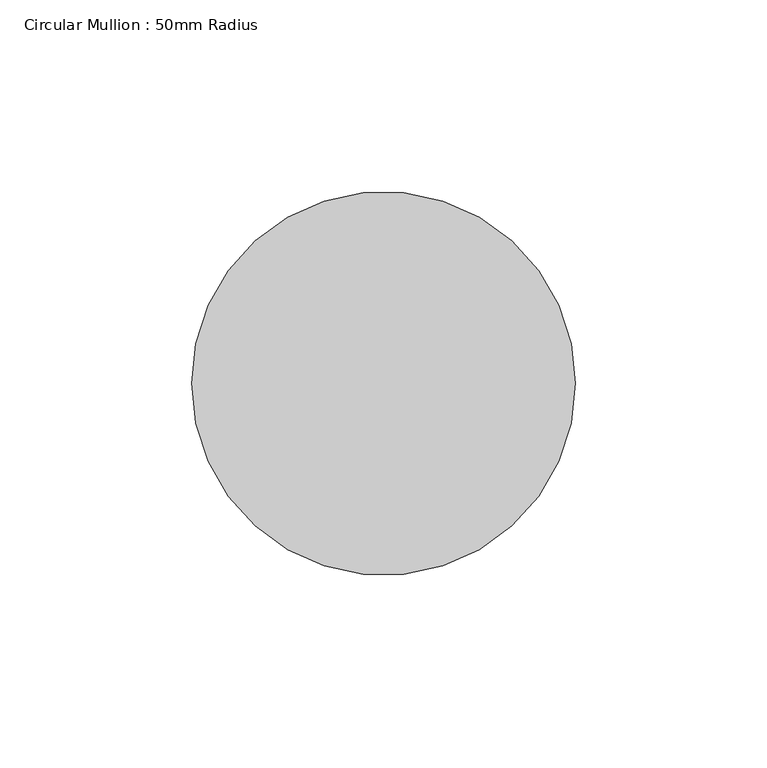
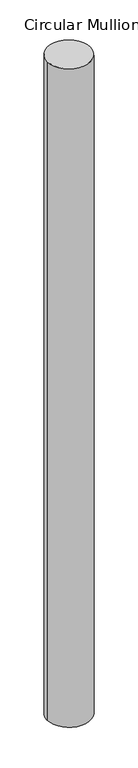
"""IFC4 building model written with IfcOpenShell, lengths in millimetres: member geometry, Circular Mullion : 50mm Radius."""

from ifc_helpers import new_model, si_unit, point, frame, origin, origin_2d, place, context, project, spatial, circle_curve, trimmed, segment, composite_curve, outline, extrude, source, transform, mapped, element, save


def circular_mullion_50mm_radius_9371b420(model_context):
    return source(origin(), model_context, "Body", "SweptSolid", [
        extrude(outline(composite_curve([segment(trimmed(circle_curve(origin_2d(), 50.0), [point((50.0, 0.0))], [point((-50.0, 0.0))], False, "CARTESIAN"), True, "CONTINUOUS"), segment(trimmed(circle_curve(origin_2d(), 50.0), [point((-50.0, 0.0))], [point((50.0, 0.0))], False, "CARTESIAN"), True, "CONTINUOUS")], self_intersect=False)), frame((0.0, 0.0, -1608.4946912), z_axis=(0.0, 0.0, 1.0), x_axis=(1.0, 0.0, 0.0)), (0.0, 0.0, 1.0), 1608.4946912),
    ])


if __name__ == "__main__":
    model = new_model("IFC4")
    model_context = context("Model", 3, world=origin())
    ifc_project = project(units=[si_unit("LENGTHUNIT", "METRE", prefix="MILLI")], contexts=[model_context])
    site = spatial("IfcSite", under=ifc_project)
    building = spatial("IfcBuilding", under=site)
    placement = place(None, origin())
    circular_mullion_50mm_radius_shape = circular_mullion_50mm_radius_9371b420(model_context)
    element("IfcMember", 1, ObjectType="Circular Mullion : 50mm Radius", at=placement, inside=building, context=model_context, shape_type="MappedRepresentation", body=[
        mapped(circular_mullion_50mm_radius_shape, transform((0.0, 0.0, 0.0), x_axis=(1.0, 0.0, 0.0), y_axis=(0.0, 1.0, 0.0), z_axis=(0.0, 0.0, 1.0))),
    ])
    save(model, "model.ifc")

# Revit data of these elements
# Type "Circular Mullion : 50mm Radius"
#   built-in parameter 1007350 = 0.164042 (stored number, unit not read)
# Element 1 (IfcMember, "Circular Mullion : 50mm Radius")
#   Materials on its faces: "Aluminium"
# Materials
#   "Aluminium": class "Metal", colour RGB 247 247 247, transparency 0, Description = "Aluminium 6061", Cost = 0
